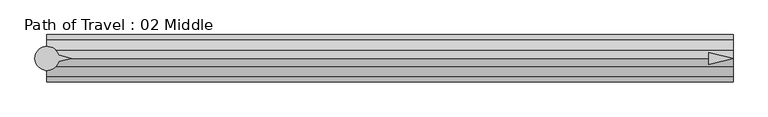
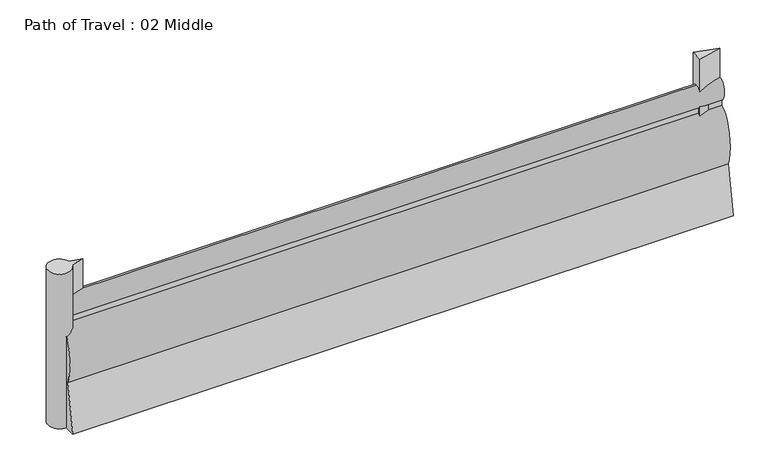
"""IFC4 building model written with IfcOpenShell, lengths in millimetres: proxy geometry, Path of Travel : 02 Middle."""

import ifcopenshell
import ifcopenshell.guid

model = None  # the IFC model being written
_history = None  # IfcOwnerHistory: only IFC2X3 demands one
_inside = {}  # id of a spatial element -> (the spatial element, [elements in it])
_under = {}  # id of a project, library or spatial element -> (it, [spatial elements below it])
_declared = {}  # id of a project -> (the project, [libraries it declares])
_typed = {}  # id of a type object -> (the type object, [elements of that type])
_made_of = {}  # id of a material, layer set ... -> (it, [elements and type objects made of it])


def new_model(schema):
    """Start an empty IFC model of exactly this schema.

    Asked for "IFC4X3", IfcOpenShell would pick the latest addendum, in which some entities
    have other attributes; the version numbers below select the first issue.
    IFC2X3 requires an IfcOwnerHistory on every rooted entity: one is made here for all.
    """
    global model, _history
    if schema == "IFC4X3":
        model = ifcopenshell.file(schema_version=(4, 3, 0, 0))
    else:
        model = ifcopenshell.file(schema=schema)
    _inside.clear()
    _under.clear()
    _declared.clear()
    _typed.clear()
    _made_of.clear()
    _history = None
    if model.schema == "IFC2X3":
        org = make("IfcOrganization", Name="unknown")
        user = make(
            "IfcPersonAndOrganization",
            ThePerson=make("IfcPerson", FamilyName="unknown"),
            TheOrganization=org,
        )
        app = make(
            "IfcApplication",
            ApplicationDeveloper=org,
            Version="unknown",
            ApplicationFullName="unknown",
            ApplicationIdentifier="unknown",
        )
        _history = make(
            "IfcOwnerHistory",
            OwningUser=user,
            OwningApplication=app,
            ChangeAction="ADDED",
            CreationDate=0,
        )
    return model


def make(cls, **values):
    """One entity of the class cls with the attributes given. An attribute that is None is left unset."""
    return model.create_entity(
        cls, **{name: value for name, value in values.items() if value is not None}
    )


def rooted(cls, **values):
    """An entity with a GlobalId (a new one), such as an element, a storey or a relation."""
    return make(cls, GlobalId=ifcopenshell.guid.new(), OwnerHistory=_history, **values)


def si_unit(unit_type, name, prefix=None):
    """IfcSIUnit, for example si_unit("LENGTHUNIT", "METRE", prefix="MILLI")."""
    return make("IfcSIUnit", UnitType=unit_type, Prefix=prefix, Name=name)


def assignment(units):
    """IfcUnitAssignment: the units of a project."""
    return None if units is None else make("IfcUnitAssignment", Units=units)


def point(xyz):
    """IfcCartesianPoint."""
    return None if xyz is None else make("IfcCartesianPoint", Coordinates=xyz)


def direction(xyz):
    """IfcDirection."""
    return None if xyz is None else make("IfcDirection", DirectionRatios=xyz)


def frame(location, z_axis=None, x_axis=None):
    """IfcAxis2Placement3D, a coordinate frame: its origin and axes. An axis left out is left unset."""
    return make(
        "IfcAxis2Placement3D",
        Location=point(location),
        Axis=direction(z_axis),
        RefDirection=direction(x_axis),
    )


def frame_2d(location, x_axis=None):
    """IfcAxis2Placement2D, a coordinate frame in the plane: its origin and x axis."""
    return make(
        "IfcAxis2Placement2D", Location=point(location), RefDirection=direction(x_axis)
    )


def origin():
    """The frame at (0, 0, 0) with its axes left unset."""
    return frame((0.0, 0.0, 0.0))


def origin_with_axes():
    """The frame at (0, 0, 0) with the z axis (0, 0, 1) and the x axis (1, 0, 0) written out."""
    return frame((0.0, 0.0, 0.0), z_axis=(0.0, 0.0, 1.0), x_axis=(1.0, 0.0, 0.0))


def place(relative_to, where):
    """IfcLocalPlacement: puts the frame where relative to a parent placement (None: the world)."""
    return make(
        "IfcLocalPlacement", PlacementRelTo=relative_to, RelativePlacement=where
    )


def context(
    kind, dimensions, precision=None, world=None, true_north=None, identifier=None
):
    """IfcGeometricRepresentationContext, for example the 3D "Model" context."""
    return make(
        "IfcGeometricRepresentationContext",
        ContextIdentifier=identifier,
        ContextType=kind,
        CoordinateSpaceDimension=dimensions,
        Precision=precision,
        WorldCoordinateSystem=world,
        TrueNorth=true_north,
    )


def project(units=None, contexts=None):
    """IfcProject with its units and contexts."""
    return rooted(
        "IfcProject",
        Name="project",
        RepresentationContexts=contexts,
        UnitsInContext=assignment(units),
    )


def spatial(cls, under=None, at=None, **own):
    """A site, building, storey or space (cls), placed at a placement, below another one or the project."""
    s = rooted(cls, ObjectPlacement=at, **own)
    if under is not None:
        _under.setdefault(under.id(), (under, []))[1].append(s)
    return s


def polyline(points):
    """IfcPolyline through the points."""
    return make("IfcPolyline", Points=[point(p) for p in points])


def circle_curve(where, radius):
    """IfcCircle in the frame where."""
    return make("IfcCircle", Position=where, Radius=radius)


def ellipse_curve(where, semi_axis1, semi_axis2):
    """IfcEllipse in the frame where."""
    return make(
        "IfcEllipse", Position=where, SemiAxis1=semi_axis1, SemiAxis2=semi_axis2
    )


def trimmed(basis, trim1, trim2, sense, master):
    """IfcTrimmedCurve: the piece of a basis curve between two trims."""
    return make(
        "IfcTrimmedCurve",
        BasisCurve=basis,
        Trim1=trim1,
        Trim2=trim2,
        SenseAgreement=sense,
        MasterRepresentation=master,
    )


def segment(curve, same_sense, transition):
    """IfcCompositeCurveSegment."""
    return make(
        "IfcCompositeCurveSegment",
        Transition=transition,
        SameSense=same_sense,
        ParentCurve=curve,
    )


def composite_curve(segments, self_intersect=None):
    """IfcCompositeCurve: segments joined end to end."""
    return make("IfcCompositeCurve", Segments=segments, SelfIntersect=self_intersect)


def outline(outer, holes=None, kind="AREA"):
    """IfcArbitraryClosedProfileDef: a profile drawn as a closed curve; with holes, ...WithVoids."""
    if holes is None:
        return make("IfcArbitraryClosedProfileDef", ProfileType=kind, OuterCurve=outer)
    return make(
        "IfcArbitraryProfileDefWithVoids",
        ProfileType=kind,
        OuterCurve=outer,
        InnerCurves=holes,
    )


def extrude(swept, where, along, depth):
    """IfcExtrudedAreaSolid: the profile swept, set in the frame where, extruded along a direction by depth."""
    return make(
        "IfcExtrudedAreaSolid",
        SweptArea=swept,
        Position=where,
        ExtrudedDirection=direction(along),
        Depth=depth,
    )


def shape(context_of_items, identifier, shape_type, items):
    """IfcShapeRepresentation: the items that make up one representation, for example the "Body"."""
    return make(
        "IfcShapeRepresentation",
        ContextOfItems=context_of_items,
        RepresentationIdentifier=identifier,
        RepresentationType=shape_type,
        Items=items,
    )


def source(mapping_origin, context_of_items, identifier, shape_type, items):
    """IfcRepresentationMap: a shape defined once, which mapped items show again and again."""
    return make(
        "IfcRepresentationMap",
        MappingOrigin=mapping_origin,
        MappedRepresentation=shape(context_of_items, identifier, shape_type, items),
    )


def transform(
    local_origin,
    x_axis=None,
    y_axis=None,
    z_axis=None,
    scale=None,
    scale2=None,
    scale3=None,
    uniform=True,
):
    """IfcCartesianTransformationOperator3D, or its non-uniform kind. x_axis, y_axis, z_axis: its Axis1, 2, 3."""
    if uniform:
        return make(
            "IfcCartesianTransformationOperator3D",
            Axis1=direction(x_axis),
            Axis2=direction(y_axis),
            LocalOrigin=point(local_origin),
            Scale=scale,
            Axis3=direction(z_axis),
        )
    return make(
        "IfcCartesianTransformationOperator3DnonUniform",
        Axis1=direction(x_axis),
        Axis2=direction(y_axis),
        LocalOrigin=point(local_origin),
        Scale=scale,
        Axis3=direction(z_axis),
        Scale2=scale2,
        Scale3=scale3,
    )


def mapped(mapping_source, mapping_target):
    """IfcMappedItem: shows the shape of a source again, moved by a transform."""
    return make(
        "IfcMappedItem", MappingSource=mapping_source, MappingTarget=mapping_target
    )


def made_of(thing, what):
    """Note that an element or type object is made of a material, layer set ...; save() writes the relation."""
    if what is not None:
        _made_of.setdefault(what.id(), (what, []))[1].append(thing)
    return thing


def element(
    cls,
    number,
    at=None,
    inside=None,
    cuts=None,
    type_object=None,
    material=None,
    context=None,
    identifier="Body",
    shape_type=None,
    held_by="IfcProductDefinitionShape",
    body=None,
    shapes=None,
    **own,
):
    """One element of the class cls, such as IfcWall. Its Tag is "e" and its number.

    at: its placement. inside: the storey or other place that contains it. cuts: it is an
    opening in that element (IfcRelVoidsElement). A single representation is given by context,
    identifier, shape_type and body (its items); several are given by shapes. held_by: the class
    of the entity that holds the representations. save() writes the other relations.
    """
    e = rooted(cls, Tag="e%d" % number, ObjectPlacement=at, **own)
    if body is not None:
        shapes = [shape(context, identifier, shape_type, body)]
    if shapes is not None:
        e.Representation = make(held_by, Representations=shapes)
    if inside is not None:
        _inside.setdefault(inside.id(), (inside, []))[1].append(e)
    if cuts is not None:
        rooted(
            "IfcRelVoidsElement", RelatingBuildingElement=cuts, RelatedOpeningElement=e
        )
    if type_object is not None:
        _typed.setdefault(type_object.id(), (type_object, []))[1].append(e)
    return made_of(e, material)


def aggregate(whole, parts):
    """IfcRelAggregates: a whole, such as a stair, and the parts it consists of."""
    return rooted("IfcRelAggregates", RelatingObject=whole, RelatedObjects=parts)


def save(model, path):
    """Write the relations noted so far, then the file.

    IfcRelAggregates (storeys below a building ...), IfcRelContainedInSpatialStructure (elements
    in a storey), IfcRelDefinesByType, IfcRelAssociatesMaterial and IfcRelDeclares: one each for
    every whole, place, type object, material and project.
    """
    for whole, parts in _under.values():
        aggregate(whole, parts)
    for where, things in _inside.values():
        rooted(
            "IfcRelContainedInSpatialStructure",
            RelatedElements=things,
            RelatingStructure=where,
        )
    for kind, things in _typed.values():
        rooted("IfcRelDefinesByType", RelatedObjects=things, RelatingType=kind)
    for what, things in _made_of.values():
        rooted("IfcRelAssociatesMaterial", RelatedObjects=things, RelatingMaterial=what)
    for by, libraries in _declared.values():
        rooted("IfcRelDeclares", RelatingContext=by, RelatedDefinitions=libraries)
    model.write(path)


def plane_surface(at):
    """IfcPlane: the flat surface through the origin of the frame at, square to its z axis."""
    return make("IfcPlane", Position=at)


def extruded_surface(curve, direction_of_extrusion, depth):
    """IfcSurfaceOfLinearExtrusion: the curve pushed along a direction by depth."""
    return make(
        "IfcSurfaceOfLinearExtrusion",
        SweptCurve=make("IfcArbitraryOpenProfileDef", ProfileType="CURVE", Curve=curve),
        ExtrudedDirection=direction(direction_of_extrusion),
        Depth=depth,
    )


def advanced_brep(points, edges, surfaces, faces):
    """IfcAdvancedBrep: a solid bounded by faces that lie on surfaces and meet in shared edges.

    An edge is (start, end): straight between two places in points (the first is 0);
    or (start, end, curve); or (start, end, curve, False) where it runs against its curve.
    A face is (place in surfaces, loops), or (place, loops, False) where it looks against
    its surface's normal. A loop lists edges by number (the first is 1), with a minus sign
    where the edge is run from its end to its start. The first loop is the outer one.
    """
    corners = [point(p) for p in points]
    vertices = [make("IfcVertexPoint", VertexGeometry=c) for c in corners]
    made = []
    for start, end, *more in edges:
        made.append(
            make(
                "IfcEdgeCurve",
                EdgeStart=vertices[start],
                EdgeEnd=vertices[end],
                EdgeGeometry=more[0] if more else make("IfcPolyline", Points=[corners[start], corners[end]]),
                SameSense=more[1] if len(more) > 1 else True,
            )
        )
    hull = []
    for where, loops, *sense in faces:
        bounds = []
        for j, loop in enumerate(loops):
            ring = [make("IfcOrientedEdge", EdgeElement=made[abs(k) - 1], Orientation=k > 0) for k in loop]
            bounds.append(
                make(
                    "IfcFaceOuterBound" if j == 0 else "IfcFaceBound",
                    Bound=make("IfcEdgeLoop", EdgeList=ring),
                    Orientation=True,
                )
            )
        hull.append(make("IfcAdvancedFace", Bounds=bounds, FaceSurface=surfaces[where], SameSense=sense[0] if sense else True))
    return make("IfcAdvancedBrep", Outer=make("IfcClosedShell", CfsFaces=hull))


def path_of_travel_02_middle_0fee29a4(model_context):
    return source(origin(), model_context, "Body", "SolidModel", [
        advanced_brep(
        [(227.5554837, 0.0, 1727.2), (227.5554837, 42.9018657, 1436.6534209), (227.5554837, 42.9018657, 1363.4763406), (227.5554837, 184.1186263, 643.4144547), (227.5554837, 297.5699544, 0.0), (227.5554837, 145.6574193, 0.0), (227.5554837, 0.0, 584.2), (227.5554837, -145.6574193, 0.0), (227.5554837, -297.5699544, 0.0), (227.5554837, -184.1186263, 643.4144547), (227.5554837, -42.9018657, 1363.4763406), (227.5554837, -42.9018657, 1436.6534209), (8834.9804837, 0.0, 1727.2), (8834.9804837, -42.9018657, 1436.6534209), (8834.9804837, -42.9018657, 1363.4763406), (8834.9804837, -184.1186263, 643.4144547), (8834.9804837, -297.5699544, 0.0), (8834.9804837, -145.6574193, 0.0), (8834.9804837, 0.0, 584.2), (8834.9804837, 145.6574193, 0.0), (8834.9804837, 297.5699544, 0.0), (8834.9804837, 184.1186263, 643.4144547), (8834.9804837, 42.9018657, 1363.4763406), (8834.9804837, 42.9018657, 1436.6534209)],
        [
            (0, 1, ellipse_curve(frame((227.5554837, 0.0, 1574.8), z_axis=(-1.0, 0.0, 0.0), x_axis=(0.0, 0.0, 1.0)), 152.4, 101.6)),
            (1, 2),
            (2, 3, ellipse_curve(frame((227.5554837, 0.0, 914.4), z_axis=(-1.0, 0.0, 0.0), x_axis=(0.0, 0.0, -1.0)), 457.2, 228.6)),
            (3, 4),
            (4, 5),
            (5, 6),
            (6, 7),
            (7, 8),
            (8, 9),
            (9, 10, ellipse_curve(frame((227.5554837, 0.0, 914.4), z_axis=(-1.0, 0.0, 0.0), x_axis=(0.0, 0.0, -1.0)), 457.2, 228.6)),
            (10, 11),
            (11, 0, ellipse_curve(frame((227.5554837, 0.0, 1574.8), z_axis=(-1.0, 0.0, 0.0), x_axis=(0.0, 0.0, 1.0)), 152.4, 101.6)),
            (12, 13, ellipse_curve(frame((8834.9804837, 0.0, 1574.8), z_axis=(1.0, 0.0, 0.0), x_axis=(0.0, 0.0, 1.0)), 152.4, 101.6)),
            (13, 14),
            (14, 15, ellipse_curve(frame((8834.9804837, 0.0, 914.4), z_axis=(1.0, 0.0, 0.0), x_axis=(0.0, 0.0, -1.0)), 457.2, 228.6)),
            (15, 16),
            (16, 17),
            (17, 18),
            (18, 19),
            (19, 20),
            (20, 21),
            (21, 22, ellipse_curve(frame((8834.9804837, 0.0, 914.4), z_axis=(1.0, 0.0, 0.0), x_axis=(0.0, 0.0, -1.0)), 457.2, 228.6)),
            (22, 23),
            (23, 12, ellipse_curve(frame((8834.9804837, 0.0, 1574.8), z_axis=(1.0, 0.0, 0.0), x_axis=(0.0, 0.0, 1.0)), 152.4, 101.6)),
            (0, 12),
            (23, 1),
            (22, 2),
            (21, 3),
            (20, 4),
            (19, 5),
            (18, 6),
            (17, 7),
            (16, 8),
            (15, 9),
            (14, 10),
            (13, 11),
        ],
        [
            plane_surface(frame((227.5554837, 0.0, 0.0), z_axis=(-1.0, 0.0, 0.0), x_axis=(0.0, 0.0, 1.0))),
            plane_surface(frame((8834.9804837, 0.0, 0.0), z_axis=(1.0, 0.0, 0.0), x_axis=(0.0, 0.0, 1.0))),
            extruded_surface(trimmed(ellipse_curve(frame((8834.9804837, 0.0, 1574.8), z_axis=(-1.0, 0.0, 0.0), x_axis=(0.0, 0.0, 1.0)), 152.4, 101.6), [point((8834.9804837, 0.0, 1727.2))], [point((8834.9804837, 42.9018657, 1436.6534209))], True, "CARTESIAN"), (-8607.425, 0.0, 0.0), 8607.425),
            plane_surface(frame((227.5554837, 42.9018657, 1436.6534209), z_axis=(0.0, 1.0, 0.0), x_axis=(1.0, 0.0, 0.0))),
            extruded_surface(trimmed(ellipse_curve(frame((8834.9804837, 0.0, 914.4), z_axis=(-1.0, 0.0, 0.0), x_axis=(0.0, 0.0, -1.0)), 457.2, 228.6), [point((8834.9804837, 42.9018657, 1363.4763406))], [point((8834.9804837, 184.1186263, 643.4144547))], True, "CARTESIAN"), (-8607.425, 0.0, 0.0), 8607.425),
            plane_surface(frame((227.5554837, 184.1186263, 643.4144547), z_axis=(0.0, 0.9848077530122078, 0.1736481776669322), x_axis=(1.0, 0.0, 0.0))),
            plane_surface(frame((227.5554837, 297.5699544, 0.0), z_axis=(0.0, 0.0, -1.0), x_axis=(1.0, 0.0, 0.0))),
            plane_surface(frame((227.5554837, 145.6574193, 0.0), z_axis=(0.0, -0.9702957262760199, -0.2419218955995739), x_axis=(1.0, 0.0, 0.0))),
            plane_surface(frame((227.5554837, 0.0, 584.2), z_axis=(0.0, 0.9702957262759961, -0.24192189559966923), x_axis=(1.0, 0.0, 0.0))),
            plane_surface(frame((227.5554837, -145.6574193, 0.0), z_axis=(0.0, 0.0, -1.0), x_axis=(1.0, 0.0, 0.0))),
            plane_surface(frame((227.5554837, -297.5699544, 0.0), z_axis=(0.0, -0.984807753012208, 0.17364817766693066), x_axis=(1.0, 0.0, 0.0))),
            extruded_surface(trimmed(ellipse_curve(frame((8834.9804837, 0.0, 914.4), z_axis=(-1.0, 0.0, 0.0), x_axis=(0.0, 0.0, -1.0)), 457.2, 228.6), [point((8834.9804837, -184.1186263, 643.4144547))], [point((8834.9804837, -42.9018657, 1363.4763406))], True, "CARTESIAN"), (-8607.425, 0.0, 0.0), 8607.425),
            plane_surface(frame((227.5554837, -42.9018657, 1363.4763406), z_axis=(0.0, -1.0, 0.0), x_axis=(1.0, 0.0, 0.0))),
            extruded_surface(trimmed(ellipse_curve(frame((8834.9804837, 0.0, 1574.8), z_axis=(-1.0, 0.0, 0.0), x_axis=(0.0, 0.0, 1.0)), 152.4, 101.6), [point((8834.9804837, -42.9018657, 1436.6534209))], [point((8834.9804837, 0.0, 1727.2))], True, "CARTESIAN"), (-8607.425, 0.0, 0.0), 8607.425),
        ],
        [
            (0, [[1, 2, 3, 4, 5, 6, 7, 8, 9, 10, 11, 12]]),
            (1, [[13, 14, 15, 16, 17, 18, 19, 20, 21, 22, 23, 24]]),
            (2, [[-1, 25, -24, 26]]),
            (3, [[-2, -26, -23, 27]]),
            (4, [[-3, -27, -22, 28]]),
            (5, [[-4, -28, -21, 29]]),
            (6, [[-5, -29, -20, 30]]),
            (7, [[-6, -30, -19, 31]]),
            (8, [[-7, -31, -18, 32]]),
            (9, [[-8, -32, -17, 33]]),
            (10, [[-9, -33, -16, 34]]),
            (11, [[-10, -34, -15, 35]]),
            (12, [[-11, -35, -14, 36]]),
            (13, [[-12, -36, -13, -25]]),
        ],
    ),
        extrude(outline(polyline([(8528.9753371, 76.2006338), (8834.9804837, 0.0), (8528.9753371, -76.2006338), (8528.9753371, 76.2006338)])), origin_with_axes(), (0.0, 0.0, 1.0), 2129.5973753),
        extrude(outline(composite_curve([segment(polyline([(372.7837828, 39.4440225), (531.182385, 0.0), (372.7837828, -39.4440225)]), True, "CONTINUOUS"), segment(trimmed(circle_curve(frame_2d((227.2200886, 0.0)), 150.8131956), [point((372.7837828, -39.4440225))], [point((372.7837828, 39.4440225))], False, "CARTESIAN"), True, "CONTINUOUS")], self_intersect=False)), origin_with_axes(), (0.0, 0.0, 1.0), 2129.5973753),
    ])


if __name__ == "__main__":
    model = new_model("IFC4")
    model_context = context("Model", 3, world=origin())
    ifc_project = project(units=[si_unit("LENGTHUNIT", "METRE", prefix="MILLI")], contexts=[model_context])
    site = spatial("IfcSite", under=ifc_project)
    building = spatial("IfcBuilding", under=site)
    placement = place(None, origin())
    path_of_travel_02_middle_shape = path_of_travel_02_middle_0fee29a4(model_context)
    element("IfcBuildingElementProxy", 1, Name="Path of Travel : 02 Middle", ObjectType="Path of Travel : 02 Middle", at=placement, inside=building, context=model_context, shape_type="MappedRepresentation", body=[
        mapped(path_of_travel_02_middle_shape, transform((0.0, 0.0, 0.0), x_axis=(1.0, 0.0, 0.0), y_axis=(0.0, 1.0, 0.0), z_axis=(0.0, 0.0, 1.0))),
    ])
    save(model, "model.ifc")

# Revit data of these elements
# Type "Path of Travel : 02 Middle"
#   Path of Egress [instance default] = 4' - 0"
#   built-in parameter 1001306 [instance default] = 4 (stored number, unit not read)
#   Dot at Start = no
#   Arrow in Middle = yes
#   Arrow at End = no
#   Egress Path = none
# Element 1 (IfcBuildingElementProxy, "Path of Travel : 02 Middle")
#   Path of Egress = 28' - 2 7/8"
#   built-in parameter 1001306 = 28.2396 (stored number, unit not read)
